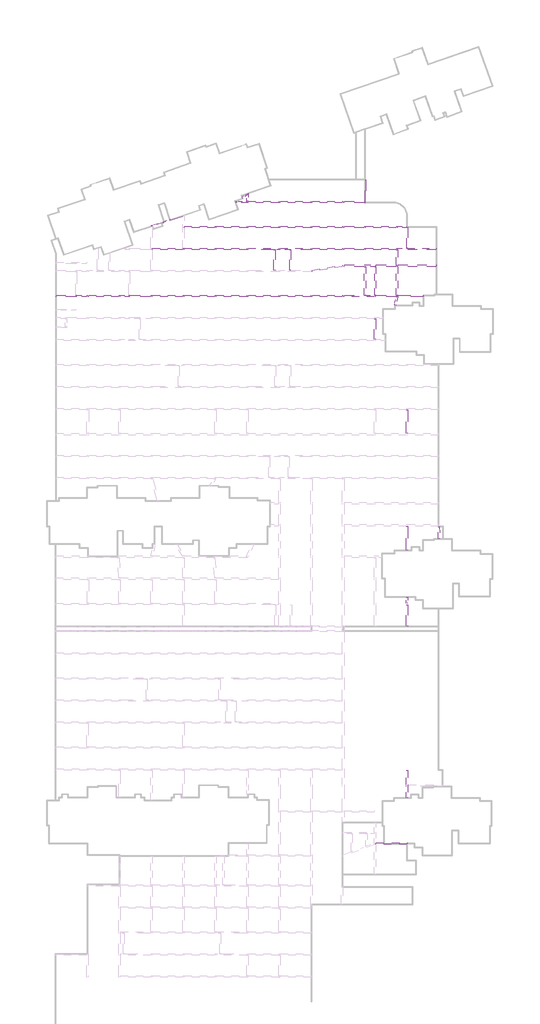
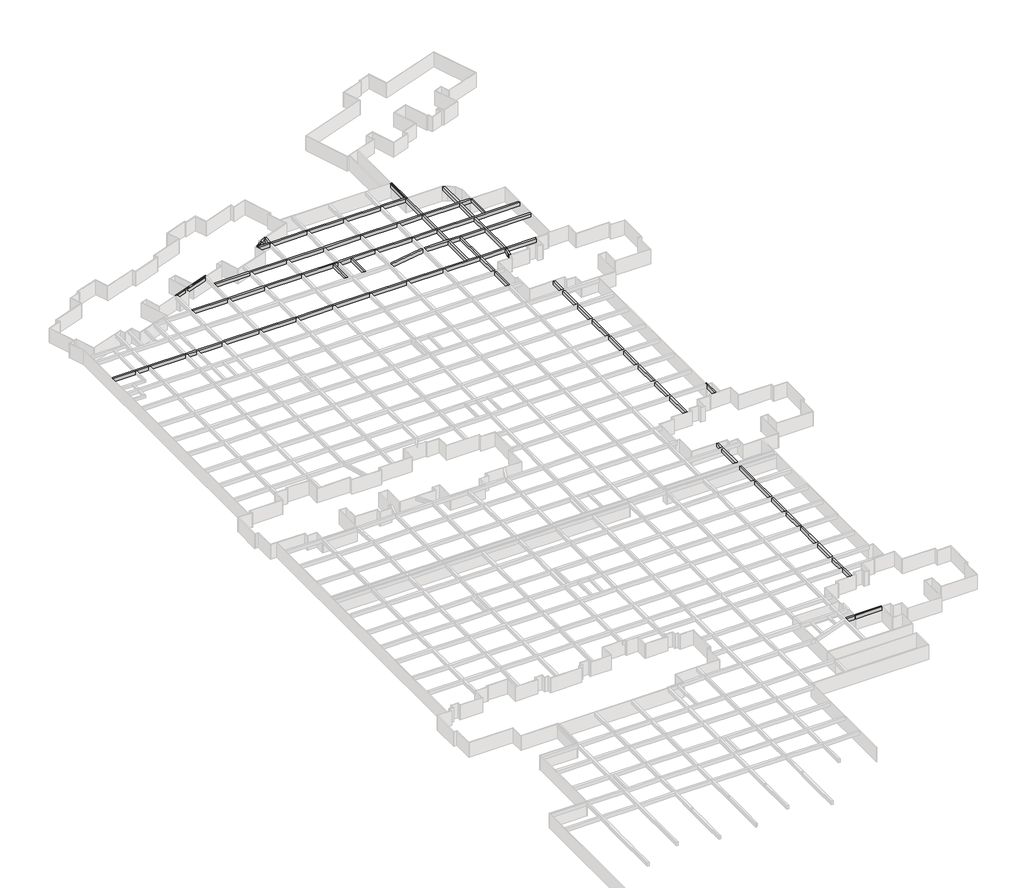
# One storey, part 14 of 14: 30 beams.
"""IFC4 building model written with IfcOpenShell, lengths in millimetres."""

from ifc_helpers import new_model, si_unit, frame, origin, place, context, project, spatial, polyline, outline, extrude, faceted_brep, element, save

model = new_model("IFC4")

# Units and contexts
model_context = context("Model", 3, world=origin())
ifc_project = project(units=[si_unit("LENGTHUNIT", "METRE", prefix="MILLI")], contexts=[model_context])

# Site, building, storey
site = spatial("IfcSite", under=ifc_project)
building = spatial("IfcBuilding", under=site)
storey = spatial("IfcBuildingStorey", under=building, Name="户型图", Elevation=0.0)

# Beams
placement = place(None, origin())
element("IfcBeam", 1, ObjectType="混凝土 - 矩形梁 : KL_beam", at=placement, inside=storey, context=model_context, shape_type="Brep", body=[
    faceted_brep([(-498755.1396851, -33759.4327531, 3300.0), (-498755.1396851, -33359.4327531, 3300.0), (-505917.6529954, -33359.4327531, 3300.0), (-506217.6529954, -33359.4327531, 3300.0), (-508367.954383, -33359.4327531, 3300.0), (-508767.954383, -33359.4327531, 3300.0), (-516417.6529954, -33359.4327531, 3300.0), (-516817.6529954, -33359.4327531, 3300.0), (-521867.6529954, -33359.4327531, 3300.0), (-522267.6529954, -33359.4327531, 3300.0), (-529867.6529954, -33359.4327531, 3300.0), (-530267.6529954, -33359.4327531, 3300.0), (-537867.6529954, -33359.4327531, 3300.0), (-538267.6529954, -33359.4327531, 3300.0), (-545867.6529954, -33359.4327531, 3300.0), (-546267.6529954, -33359.4327531, 3300.0), (-553867.6529954, -33359.4327531, 3300.0), (-554267.6529954, -33359.4327531, 3300.0), (-561867.6529954, -33359.4327531, 3300.0), (-562267.6529954, -33359.4327531, 3300.0), (-569867.6529954, -33359.4327531, 3300.0), (-569867.6529954, -33759.4327531, 3300.0), (-562267.6529954, -33759.4327531, 3300.0), (-561867.6529954, -33759.4327531, 3300.0), (-554267.6529954, -33759.4327531, 3300.0), (-553867.6529954, -33759.4327531, 3300.0), (-546267.6529954, -33759.4327531, 3300.0), (-545867.6529954, -33759.4327531, 3300.0), (-539417.6529954, -33759.4327531, 3300.0), (-539117.6529954, -33759.4327531, 3300.0), (-538267.6529954, -33759.4327531, 3300.0), (-537867.6529954, -33759.4327531, 3300.0), (-535517.6529954, -33759.4327531, 3300.0), (-535217.6529954, -33759.4327531, 3300.0), (-530267.6529954, -33759.4327531, 3300.0), (-529867.6529954, -33759.4327531, 3300.0), (-522267.6529954, -33759.4327531, 3300.0), (-521867.6529954, -33759.4327531, 3300.0), (-516817.6529954, -33759.4327531, 3300.0), (-516417.6529954, -33759.4327531, 3300.0), (-508767.954383, -33759.4327531, 3300.0), (-508367.954383, -33759.4327531, 3300.0), (-498755.1396851, -33759.4327531, 2500.0), (-569867.6529954, -33759.4327531, 2500.0), (-562267.6529954, -33759.4327531, 2500.0), (-561867.6529954, -33759.4327531, 2500.0), (-554267.6529954, -33759.4327531, 2500.0), (-553867.6529954, -33759.4327531, 2500.0), (-546267.6529954, -33759.4327531, 2500.0), (-545867.6529954, -33759.4327531, 2500.0), (-538267.6529954, -33759.4327531, 2500.0), (-537867.6529954, -33759.4327531, 2500.0), (-530267.6529954, -33759.4327531, 2500.0), (-529867.6529954, -33759.4327531, 2500.0), (-522267.6529954, -33759.4327531, 2500.0), (-521867.6529954, -33759.4327531, 2500.0), (-516817.6529954, -33759.4327531, 2500.0), (-516417.6529954, -33759.4327531, 2500.0), (-508767.954383, -33759.4327531, 2500.0), (-508367.954383, -33759.4327531, 2500.0), (-498755.1396851, -33359.4327531, 2500.0), (-569867.6529954, -33359.4327531, 2500.0), (-562267.6529954, -33359.4327531, 2500.0), (-561867.6529954, -33359.4327531, 2500.0), (-554267.6529954, -33359.4327531, 2500.0), (-553867.6529954, -33359.4327531, 2500.0), (-546267.6529954, -33359.4327531, 2500.0), (-545867.6529954, -33359.4327531, 2500.0), (-538267.6529954, -33359.4327531, 2500.0), (-537867.6529954, -33359.4327531, 2500.0), (-530267.6529954, -33359.4327531, 2500.0), (-529867.6529954, -33359.4327531, 2500.0), (-522267.6529954, -33359.4327531, 2500.0), (-521867.6529954, -33359.4327531, 2500.0), (-516817.6529954, -33359.4327531, 2500.0), (-516417.6529954, -33359.4327531, 2500.0), (-508767.954383, -33359.4327531, 2500.0), (-508367.954383, -33359.4327531, 2500.0)], [[[0, 1, 2, 3, 4, 5, 6, 7, 8, 9, 10, 11, 12, 13, 14, 15, 16, 17, 18, 19, 20, 21, 22, 23, 24, 25, 26, 27, 28, 29, 30, 31, 32, 33, 34, 35, 36, 37, 38, 39, 40, 41]], [[42, 0, 41, 40, 39, 38, 37, 36, 35, 34, 33, 32, 31, 30, 29, 28, 27, 26, 25, 24, 23, 22, 21, 43, 44, 45, 46, 47, 48, 49, 50, 51, 52, 53, 54, 55, 56, 57, 58, 59]], [[60, 42, 59, 58, 57, 56, 55, 54, 53, 52, 51, 50, 49, 48, 47, 46, 45, 44, 43, 61, 62, 63, 64, 65, 66, 67, 68, 69, 70, 71, 72, 73, 74, 75, 76, 77]], [[1, 60, 77, 76, 75, 74, 73, 72, 71, 70, 69, 68, 67, 66, 65, 64, 63, 62, 61, 20, 19, 18, 17, 16, 15, 14, 13, 12, 11, 10, 9, 8, 7, 6, 5, 4, 3, 2]], [[1, 0, 42, 60]], [[21, 20, 61, 43]]]),
])
element("IfcBeam", 2, ObjectType="混凝土 - 矩形梁 : KL_beam", at=placement, inside=storey, context=model_context, shape_type="Brep", body=[
    faceted_brep([(-506067.6529954, -28259.4327531, 3300.0), (-506067.6529954, -28059.4327531, 3300.0), (-506155.1396851, -28059.4327531, 3300.0), (-506155.1396851, -27939.4327531, 3300.0), (-506155.1396851, -27859.4327531, 3300.0), (-508367.954383, -27859.4327531, 3300.0), (-508767.954383, -27859.4327531, 3300.0), (-516417.6529954, -27859.4327531, 3300.0), (-516817.6529954, -27859.4327531, 3300.0), (-521867.6529954, -27859.4327531, 3300.0), (-522267.6529954, -27859.4327531, 3300.0), (-529867.6529954, -27859.4327531, 3300.0), (-530267.6529954, -27859.4327531, 3300.0), (-537867.6529954, -27859.4327531, 3300.0), (-538267.6529954, -27859.4327531, 3300.0), (-545867.6529954, -27859.4327531, 3300.0), (-546267.6529954, -27859.4327531, 3300.0), (-553867.6529954, -27859.4327531, 3300.0), (-554267.6529954, -27859.4327531, 3300.0), (-561867.6529954, -27859.4327531, 3300.0), (-561867.6529954, -28259.4327531, 3300.0), (-554267.6529954, -28259.4327531, 3300.0), (-553867.6529954, -28259.4327531, 3300.0), (-546267.6529954, -28259.4327531, 3300.0), (-545867.6529954, -28259.4327531, 3300.0), (-538267.6529954, -28259.4327531, 3300.0), (-537867.6529954, -28259.4327531, 3300.0), (-530267.6529954, -28259.4327531, 3300.0), (-529867.6529954, -28259.4327531, 3300.0), (-522267.6529954, -28259.4327531, 3300.0), (-521867.6529954, -28259.4327531, 3300.0), (-516817.6529954, -28259.4327531, 3300.0), (-516417.6529954, -28259.4327531, 3300.0), (-508767.954383, -28259.4327531, 3300.0), (-508367.954383, -28259.4327531, 3300.0), (-506217.6529954, -28259.4327531, 3300.0), (-506067.6529954, -28259.4327531, 2500.0), (-506067.6529954, -28259.4327531, 2700.0), (-561867.6529954, -28259.4327531, 2500.0), (-554267.6529954, -28259.4327531, 2500.0), (-553867.6529954, -28259.4327531, 2500.0), (-546267.6529954, -28259.4327531, 2500.0), (-545867.6529954, -28259.4327531, 2500.0), (-538267.6529954, -28259.4327531, 2500.0), (-537867.6529954, -28259.4327531, 2500.0), (-530267.6529954, -28259.4327531, 2500.0), (-529867.6529954, -28259.4327531, 2500.0), (-522267.6529954, -28259.4327531, 2500.0), (-521867.6529954, -28259.4327531, 2500.0), (-516817.6529954, -28259.4327531, 2500.0), (-516417.6529954, -28259.4327531, 2500.0), (-508767.954383, -28259.4327531, 2500.0), (-508367.954383, -28259.4327531, 2500.0), (-506067.6529954, -28059.4327531, 2500.0), (-561867.6529954, -27859.4327531, 2500.0), (-554267.6529954, -27859.4327531, 2500.0), (-553867.6529954, -27859.4327531, 2500.0), (-546267.6529954, -27859.4327531, 2500.0), (-545867.6529954, -27859.4327531, 2500.0), (-538267.6529954, -27859.4327531, 2500.0), (-537867.6529954, -27859.4327531, 2500.0), (-530267.6529954, -27859.4327531, 2500.0), (-529867.6529954, -27859.4327531, 2500.0), (-522267.6529954, -27859.4327531, 2500.0), (-521867.6529954, -27859.4327531, 2500.0), (-516817.6529954, -27859.4327531, 2500.0), (-516417.6529954, -27859.4327531, 2500.0), (-508767.954383, -27859.4327531, 2500.0), (-508367.954383, -27859.4327531, 2500.0), (-506155.1396851, -27859.4327531, 2500.0), (-506155.1396851, -28059.4327531, 2500.0), (-506067.6529954, -28059.4327531, 2700.0)], [[[0, 1, 2, 3, 4, 5, 6, 7, 8, 9, 10, 11, 12, 13, 14, 15, 16, 17, 18, 19, 20, 21, 22, 23, 24, 25, 26, 27, 28, 29, 30, 31, 32, 33, 34, 35]], [[36, 37, 0, 35, 34, 33, 32, 31, 30, 29, 28, 27, 26, 25, 24, 23, 22, 21, 20, 38, 39, 40, 41, 42, 43, 44, 45, 46, 47, 48, 49, 50, 51, 52]], [[53, 36, 52, 51, 50, 49, 48, 47, 46, 45, 44, 43, 42, 41, 40, 39, 38, 54, 55, 56, 57, 58, 59, 60, 61, 62, 63, 64, 65, 66, 67, 68, 69, 70]], [[4, 69, 68, 67, 66, 65, 64, 63, 62, 61, 60, 59, 58, 57, 56, 55, 54, 19, 18, 17, 16, 15, 14, 13, 12, 11, 10, 9, 8, 7, 6, 5]], [[70, 2, 1, 71, 53]], [[2, 70, 69, 4, 3]], [[0, 37, 36, 53, 71, 1]], [[20, 19, 54, 38]]]),
])
element("IfcBeam", 3, ObjectType="混凝土 - 矩形梁 : KL_beam", at=placement, inside=storey, context=model_context, shape_type="Brep", body=[
    faceted_brep([(-516677.6529954, -21959.2569935, 3300.0), (-516677.6529954, -21839.2569935, 3300.0), (-516677.6529954, -21559.4327531, 3300.0), (-516817.6529954, -21559.4327531, 3300.0), (-521867.6529954, -21559.4327531, 3300.0), (-522267.6529954, -21559.4327531, 3300.0), (-529867.6529954, -21559.4327531, 3300.0), (-530267.6529954, -21559.4327531, 3300.0), (-537867.6529954, -21559.4327531, 3300.0), (-538267.6529954, -21559.4327531, 3300.0), (-545867.6529954, -21559.4327531, 3300.0), (-546267.6529954, -21559.4327531, 3300.0), (-546267.6529954, -21959.4327531, 3300.0), (-545867.6529954, -21959.4327531, 3300.0), (-538267.6529954, -21959.4327531, 3300.0), (-537867.6529954, -21959.4327531, 3300.0), (-530267.6529954, -21959.4327531, 3300.0), (-529867.6529954, -21959.4327531, 3300.0), (-522267.6529954, -21959.4327531, 3300.0), (-521867.6529954, -21959.4327531, 3300.0), (-516817.6529954, -21959.4327531, 3300.0), (-516557.6529954, -21959.4327531, 3300.0), (-516557.6529954, -21959.2569935, 3300.0), (-516557.6529954, -21959.4327531, 2500.0), (-546267.6529954, -21959.4327531, 2500.0), (-545867.6529954, -21959.4327531, 2500.0), (-538267.6529954, -21959.4327531, 2500.0), (-537867.6529954, -21959.4327531, 2500.0), (-530267.6529954, -21959.4327531, 2500.0), (-529867.6529954, -21959.4327531, 2500.0), (-522267.6529954, -21959.4327531, 2500.0), (-521867.6529954, -21959.4327531, 2500.0), (-516817.6529954, -21959.4327531, 2500.0), (-516677.6529954, -21559.4327531, 2500.0), (-516677.6529954, -21959.2569935, 2500.0), (-516557.6529954, -21959.2569935, 2500.0), (-546267.6529954, -21559.4327531, 2500.0), (-545867.6529954, -21559.4327531, 2500.0), (-538267.6529954, -21559.4327531, 2500.0), (-537867.6529954, -21559.4327531, 2500.0), (-530267.6529954, -21559.4327531, 2500.0), (-529867.6529954, -21559.4327531, 2500.0), (-522267.6529954, -21559.4327531, 2500.0), (-521867.6529954, -21559.4327531, 2500.0), (-516817.6529954, -21559.4327531, 2500.0)], [[[0, 1, 2, 3, 4, 5, 6, 7, 8, 9, 10, 11, 12, 13, 14, 15, 16, 17, 18, 19, 20, 21, 22]], [[23, 21, 20, 19, 18, 17, 16, 15, 14, 13, 12, 24, 25, 26, 27, 28, 29, 30, 31, 32]], [[33, 34, 35, 23, 32, 31, 30, 29, 28, 27, 26, 25, 24, 36, 37, 38, 39, 40, 41, 42, 43, 44]], [[2, 33, 44, 43, 42, 41, 40, 39, 38, 37, 36, 11, 10, 9, 8, 7, 6, 5, 4, 3]], [[21, 23, 35, 22]], [[0, 34, 33, 2, 1]], [[34, 0, 22, 35]], [[12, 11, 36, 24]]]),
])
element("IfcBeam", 4, ObjectType="混凝土 - 矩形梁 : KL_beam", at=placement, inside=storey, context=model_context, shape_type="SweptSolid", body=[
    extrude(outline(polyline([(-529867.6529954, -39229.5561723), (-529867.6529954, -38824.309334), (-522267.6529954, -37589.309334), (-522267.6529954, -37994.5561723), (-529867.6529954, -39229.5561723)])), frame((0.0, 0.0, 2500.0), z_axis=(0.0, 0.0, 1.0), x_axis=(1.0, 0.0, 0.0)), (0.0, 0.0, 1.0), 800.0),
])
element("IfcBeam", 5, ObjectType="混凝土 - 矩形梁 : KL_beam", at=placement, inside=storey, context=model_context, shape_type="Brep", body=[
    faceted_brep([(-521867.6529954, -37559.4327532, 3300.0), (-521867.6529954, -37959.4327532, 3300.0), (-516817.6529954, -37959.4327532, 3300.0), (-516417.6529954, -37959.4327532, 3300.0), (-514217.6529954, -37959.4327532, 3300.0), (-513917.6529954, -37959.4327532, 3300.0), (-513917.6529954, -37559.4327532, 3300.0), (-516417.6529954, -37559.4327532, 3300.0), (-516817.6529954, -37559.4327532, 3300.0), (-513917.6529954, -37959.4327532, 2500.0), (-513917.6529954, -37959.4327532, 2700.0), (-521867.6529954, -37959.4327532, 2500.0), (-516817.6529954, -37959.4327532, 2500.0), (-516417.6529954, -37959.4327532, 2500.0), (-521867.6529954, -37559.4327532, 2500.0), (-516817.6529954, -37559.4327532, 2500.0), (-516417.6529954, -37559.4327532, 2500.0), (-513917.6529954, -37559.4327532, 2500.0)], [[[0, 1, 2, 3, 4, 5, 6, 7, 8]], [[9, 10, 5, 4, 3, 2, 1, 11, 12, 13]], [[11, 14, 15, 16, 17, 9, 13, 12]], [[14, 0, 8, 7, 6, 17, 16, 15]], [[0, 14, 11, 1]], [[6, 5, 10, 9, 17]]]),
])
element("IfcBeam", 6, ObjectType="混凝土 - 矩形梁 : KL_beam", at=placement, inside=storey, context=model_context, shape_type="SweptSolid", body=[
    extrude(outline(polyline([(-513917.6529954, -37959.4327532), (-513917.6529954, -37559.4327532), (-508767.954383, -37559.4327532), (-508767.954383, -37959.4327532), (-513917.6529954, -37959.4327532)])), frame((0.0, 0.0, 2500.0), z_axis=(0.0, 0.0, 1.0), x_axis=(1.0, 0.0, 0.0)), (0.0, 0.0, 1.0), 800.0),
])
element("IfcBeam", 7, ObjectType="混凝土 - 矩形梁 : KL_beam", at=placement, inside=storey, context=model_context, shape_type="SweptSolid", body=[
    extrude(outline(polyline([(-498755.1396851, -37559.4327532), (-498755.1396851, -37959.4327532), (-508367.954383, -37959.4327532), (-508367.954383, -37559.4327532), (-498755.1396851, -37559.4327532)])), frame((0.0, 0.0, 2500.0), z_axis=(0.0, 0.0, 1.0), x_axis=(1.0, 0.0, 0.0)), (0.0, 0.0, 1.0), 800.0),
])
element("IfcBeam", 8, ObjectType="混凝土 - 矩形梁 : KL_beam", at=placement, inside=storey, context=model_context, shape_type="Brep", body=[
    faceted_brep([(-508367.954383, -45559.4327531, 3300.0), (-508367.954383, -45159.4327531, 3300.0), (-508767.954383, -45159.4327531, 3300.0), (-513917.6529954, -45159.4327531, 3300.0), (-514217.6529954, -45159.4327531, 3300.0), (-516417.6529954, -45159.4327531, 3300.0), (-516817.6529954, -45159.4327531, 3300.0), (-521867.6529954, -45159.4327531, 3300.0), (-522267.6529954, -45159.4327531, 3300.0), (-529867.6529954, -45159.4327531, 3300.0), (-530267.6529954, -45159.4327531, 3300.0), (-537867.6529954, -45159.4327531, 3300.0), (-538267.6529954, -45159.4327531, 3300.0), (-545867.6529954, -45159.4327531, 3300.0), (-546267.6529954, -45159.4327531, 3300.0), (-553867.6529954, -45159.4327531, 3300.0), (-554267.6529954, -45159.4327531, 3300.0), (-561867.6529954, -45159.4327531, 3300.0), (-562267.6529954, -45159.4327531, 3300.0), (-569867.6529954, -45159.4327531, 3300.0), (-570267.6529954, -45159.4327531, 3300.0), (-575517.6529954, -45159.4327531, 3300.0), (-575817.6529954, -45159.4327531, 3300.0), (-577867.6529954, -45159.4327531, 3300.0), (-578267.6529954, -45159.4327531, 3300.0), (-585867.6529954, -45159.4327531, 3300.0), (-586267.6529954, -45159.4327531, 3300.0), (-588817.6529954, -45159.4327531, 3300.0), (-589117.6529954, -45159.4327531, 3300.0), (-594019.2557706, -45159.4327531, 3300.0), (-594019.2557706, -45559.4327531, 3300.0), (-589117.6529954, -45559.4327531, 3300.0), (-588817.6529954, -45559.4327531, 3300.0), (-586267.6529954, -45559.4327531, 3300.0), (-585867.6529954, -45559.4327531, 3300.0), (-578267.6529954, -45559.4327531, 3300.0), (-577867.6529954, -45559.4327531, 3300.0), (-575817.6529954, -45559.4327531, 3300.0), (-575517.6529954, -45559.4327531, 3300.0), (-570267.6529954, -45559.4327531, 3300.0), (-569867.6529954, -45559.4327531, 3300.0), (-562267.6529954, -45559.4327531, 3300.0), (-561867.6529954, -45559.4327531, 3300.0), (-554267.6529954, -45559.4327531, 3300.0), (-553867.6529954, -45559.4327531, 3300.0), (-546267.6529954, -45559.4327531, 3300.0), (-545867.6529954, -45559.4327531, 3300.0), (-538267.6529954, -45559.4327531, 3300.0), (-537867.6529954, -45559.4327531, 3300.0), (-530267.6529954, -45559.4327531, 3300.0), (-529867.6529954, -45559.4327531, 3300.0), (-522267.6529954, -45559.4327531, 3300.0), (-521867.6529954, -45559.4327531, 3300.0), (-514267.6529954, -45559.4327531, 3300.0), (-513867.6529954, -45559.4327531, 3300.0), (-508813.169158, -45559.4327531, 3300.0), (-508404.6952544, -45559.4327531, 3300.0), (-508367.954383, -45559.4327531, 2500.0), (-594019.2557706, -45559.4327531, 2500.0), (-586267.6529954, -45559.4327531, 2500.0), (-585867.6529954, -45559.4327531, 2500.0), (-578267.6529954, -45559.4327531, 2500.0), (-577867.6529954, -45559.4327531, 2500.0), (-570267.6529954, -45559.4327531, 2500.0), (-569867.6529954, -45559.4327531, 2500.0), (-562267.6529954, -45559.4327531, 2500.0), (-561867.6529954, -45559.4327531, 2500.0), (-554267.6529954, -45559.4327531, 2500.0), (-553867.6529954, -45559.4327531, 2500.0), (-546267.6529954, -45559.4327531, 2500.0), (-545867.6529954, -45559.4327531, 2500.0), (-538267.6529954, -45559.4327531, 2500.0), (-537867.6529954, -45559.4327531, 2500.0), (-530267.6529954, -45559.4327531, 2500.0), (-529867.6529954, -45559.4327531, 2500.0), (-522267.6529954, -45559.4327531, 2500.0), (-521867.6529954, -45559.4327531, 2500.0), (-514267.6529954, -45559.4327531, 2500.0), (-513867.6529954, -45559.4327531, 2500.0), (-508813.169158, -45559.4327531, 2500.0), (-508404.6952544, -45559.4327531, 2500.0), (-508367.954383, -45159.4327531, 2500.0), (-594019.2557706, -45159.4327531, 2500.0), (-586267.6529954, -45159.4327531, 2500.0), (-585867.6529954, -45159.4327531, 2500.0), (-578267.6529954, -45159.4327531, 2500.0), (-577867.6529954, -45159.4327531, 2500.0), (-570267.6529954, -45159.4327531, 2500.0), (-569867.6529954, -45159.4327531, 2500.0), (-562267.6529954, -45159.4327531, 2500.0), (-561867.6529954, -45159.4327531, 2500.0), (-554267.6529954, -45159.4327531, 2500.0), (-553867.6529954, -45159.4327531, 2500.0), (-546267.6529954, -45159.4327531, 2500.0), (-545867.6529954, -45159.4327531, 2500.0), (-538267.6529954, -45159.4327531, 2500.0), (-537867.6529954, -45159.4327531, 2500.0), (-530267.6529954, -45159.4327531, 2500.0), (-529867.6529954, -45159.4327531, 2500.0), (-522267.6529954, -45159.4327531, 2500.0), (-521867.6529954, -45159.4327531, 2500.0), (-516817.6529954, -45159.4327531, 2500.0), (-516417.6529954, -45159.4327531, 2500.0), (-508767.954383, -45159.4327531, 2500.0)], [[[0, 1, 2, 3, 4, 5, 6, 7, 8, 9, 10, 11, 12, 13, 14, 15, 16, 17, 18, 19, 20, 21, 22, 23, 24, 25, 26, 27, 28, 29, 30, 31, 32, 33, 34, 35, 36, 37, 38, 39, 40, 41, 42, 43, 44, 45, 46, 47, 48, 49, 50, 51, 52, 53, 54, 55, 56]], [[57, 0, 56, 55, 54, 53, 52, 51, 50, 49, 48, 47, 46, 45, 44, 43, 42, 41, 40, 39, 38, 37, 36, 35, 34, 33, 32, 31, 30, 58, 59, 60, 61, 62, 63, 64, 65, 66, 67, 68, 69, 70, 71, 72, 73, 74, 75, 76, 77, 78, 79, 80]], [[81, 57, 80, 79, 78, 77, 76, 75, 74, 73, 72, 71, 70, 69, 68, 67, 66, 65, 64, 63, 62, 61, 60, 59, 58, 82, 83, 84, 85, 86, 87, 88, 89, 90, 91, 92, 93, 94, 95, 96, 97, 98, 99, 100, 101, 102, 103]], [[1, 81, 103, 102, 101, 100, 99, 98, 97, 96, 95, 94, 93, 92, 91, 90, 89, 88, 87, 86, 85, 84, 83, 82, 29, 28, 27, 26, 25, 24, 23, 22, 21, 20, 19, 18, 17, 16, 15, 14, 13, 12, 11, 10, 9, 8, 7, 6, 5, 4, 3, 2]], [[30, 29, 82, 58]], [[1, 0, 57, 81]]]),
])
element("IfcBeam", 9, ObjectType="混凝土 - 矩形梁 : KL_beam", at=placement, inside=storey, context=model_context, shape_type="Brep", body=[
    faceted_brep([(-502015.1396851, -45559.4327531, 3300.0), (-502015.1396851, -45292.3075196, 3300.0), (-502015.1396851, -45172.3075196, 3300.0), (-501895.1396851, -45172.3075196, 3300.0), (-501895.1396851, -45159.4327531, 3300.0), (-508367.954383, -45159.4327531, 3300.0), (-508367.954383, -45559.4327531, 3300.0), (-502015.1396851, -45559.4327531, 2500.0), (-508367.954383, -45559.4327531, 2500.0), (-502015.1396851, -45172.3075196, 2500.0), (-508367.954383, -45159.4327531, 2500.0), (-501895.1396851, -45159.4327531, 2500.0), (-501895.1396851, -45172.3075196, 2500.0)], [[[0, 1, 2, 3, 4, 5, 6]], [[7, 0, 6, 8]], [[9, 7, 8, 10, 11, 12]], [[4, 11, 10, 5]], [[11, 4, 3, 12]], [[0, 7, 9, 2, 1]], [[2, 9, 12, 3]], [[6, 5, 10, 8]]]),
])
element("IfcBeam", 10, ObjectType="混凝土 - 矩形梁 : KL_beam", at=placement, inside=storey, context=model_context, shape_type="Brep", body=[
    faceted_brep([(-567194.1270285, -27105.5852075, 2500.0), (-567194.1270285, -27105.5852075, 3300.0), (-567238.9034733, -26972.9387979, 3300.0), (-567238.9034733, -26972.9387979, 2500.0), (-562267.6529954, -25442.5926439, 2500.0), (-562267.6529954, -25442.5926439, 3300.0), (-562267.6529954, -25294.8313886, 2500.0), (-562267.6529954, -25294.8313886, 3300.0), (-566850.6148569, -26841.8671476, 3300.0), (-566850.6148569, -26841.8671476, 2500.0), (-566888.9946667, -26728.170225, 3300.0), (-566933.7711116, -26595.5238154, 3300.0), (-566933.7711116, -26595.5238154, 2500.0), (-565497.231347, -26385.0157164, 3300.0), (-565497.231347, -26385.0157164, 2500.0), (-565580.3876017, -26138.6723843, 2500.0), (-565580.3876017, -26138.6723843, 3300.0), (-565383.5344245, -26346.6359066, 3300.0)], [[[0, 1, 2, 3]], [[1, 0, 4, 5]], [[5, 4, 6, 7]], [[8, 9, 3, 2]], [[9, 8, 10, 11, 12]], [[13, 14, 15, 16]], [[14, 13, 17, 7, 6]], [[12, 11, 16, 15]], [[1, 5, 7, 17, 13, 16, 11, 10, 8, 2]], [[4, 0, 3, 9, 12, 15, 14, 6]]]),
    faceted_brep([(-565421.9142343, -26232.938984, 3300.0), (-561948.5420308, -25060.4590103, 3300.0), (-561993.3184757, -24927.8126006, 3300.0), (-565466.6906792, -26100.2925744, 3300.0), (-561993.3184757, -24927.8126006, 2500.0), (-561948.5420308, -25060.4590103, 2500.0), (-565421.9142343, -26232.938984, 2500.0), (-565466.6906792, -26100.2925744, 2500.0)], [[[0, 1, 2, 3]], [[4, 5, 6, 7]], [[2, 4, 7, 3]], [[4, 2, 1, 5]], [[0, 6, 5, 1]], [[3, 7, 6, 0]]]),
    faceted_brep([(-567277.2832832, -26859.2418753, 3300.0), (-567277.2832832, -26859.2418753, 2500.0), (-567002.6915893, -26766.5500349, 2500.0), (-567002.6915893, -26766.5500349, 3300.0), (-567322.059728, -26726.5954657, 3300.0), (-567322.059728, -26726.5954657, 2500.0), (-567047.4680341, -26633.9036253, 3300.0), (-567047.4680341, -26633.9036253, 2500.0)], [[[0, 1, 2, 3]], [[4, 5, 1, 0]], [[6, 3, 2, 7]], [[4, 0, 3, 6]], [[1, 5, 7, 2]], [[5, 4, 6, 7]]]),
])
element("IfcBeam", 11, ObjectType="混凝土 - 矩形梁 : KL_beam", at=placement, inside=storey, context=model_context, shape_type="SweptSolid", body=[
    extrude(outline(polyline([(-570131.0843915, -27668.6081906), (-566657.7255059, -26503.8089794), (-566575.5004889, -26748.998872), (-566850.6148569, -26841.8671476), (-566888.9946667, -26728.170225), (-567665.8108881, -26990.3941992), (-567627.6568009, -27104.1673172), (-569867.6529954, -27860.3058838), (-569867.6529954, -27798.4711532), (-570060.5174914, -27798.4711532), (-570084.8033221, -27806.6154647), (-570131.0843915, -27668.6081906)])), frame((0.0, 0.0, 2500.0), z_axis=(0.0, 0.0, 1.0), x_axis=(1.0, 0.0, 0.0)), (0.0, 0.0, 1.0), 800.0),
])
element("IfcBeam", 12, ObjectType="混凝土 - 矩形梁 : KL_beam", at=placement, inside=storey, context=model_context, shape_type="Brep", body=[
    faceted_brep([(-546179.2460997, -19597.0204925, 2500.0), (-546179.2460997, -19597.0204925, 3300.0), (-546161.9464573, -19622.8510562, 3300.0), (-546161.9464573, -19622.8510562, 2500.0), (-546273.8443347, -19660.3762771, 3300.0), (-546273.8443347, -19660.3762771, 2500.0)], [[[0, 1, 2, 3]], [[2, 1, 4]], [[0, 3, 5]], [[1, 0, 5, 4]], [[3, 2, 4, 5]]]),
    faceted_brep([(-548829.2329536, -21853.2325756, 2500.0), (-548829.2329536, -21853.2325756, 3300.0), (-549026.0010884, -21559.4327531, 3300.0), (-549029.1521409, -21554.7278314, 3300.0), (-549029.1521409, -21554.7278314, 2500.0), (-549026.0010884, -21559.4327531, 2500.0), (-548390.5524947, -21559.4327531, 2500.0), (-547736.0310301, -21121.0765735, 2500.0), (-547736.0310301, -21121.0765735, 3300.0), (-548390.5524947, -21559.4327531, 3300.0)], [[[0, 1, 2, 3, 4, 5]], [[1, 0, 6, 7, 8, 9]], [[4, 3, 8, 7]], [[3, 2, 1, 9, 8]], [[0, 5, 4, 7, 6]]]),
    faceted_brep([(-545956.6604485, -19929.3691466, 2500.0), (-545956.6604485, -19929.3691466, 3300.0), (-546267.6529954, -20137.6518572, 3300.0), (-547255.5675769, -20799.2932016, 3300.0), (-547255.5675769, -20799.2932016, 2500.0), (-546267.6529954, -20137.6518572, 2500.0), (-547388.1122393, -20406.640912, 3300.0), (-547388.1122393, -20406.640912, 2500.0), (-546092.7261364, -19726.205789, 3300.0), (-546092.7261364, -19726.205789, 2500.0), (-546652.3562174, -19913.8790754, 2500.0), (-546652.3562174, -19913.8790754, 3300.0)], [[[0, 1, 2, 3, 4, 5]], [[3, 6, 7, 4]], [[8, 9, 10, 11]], [[1, 0, 9, 8]], [[3, 2, 1, 8, 11, 6]], [[0, 5, 4, 7, 10, 9]], [[7, 6, 11, 10]]]),
    faceted_brep([(-547491.4111778, -20475.8238654, 3300.0), (-547359.0031341, -20868.0714336, 3300.0), (-547359.0031341, -20868.0714336, 2500.0), (-547491.4111778, -20475.8238654, 2500.0), (-548797.2519129, -21350.3916022, 3300.0), (-548797.2519129, -21350.3916022, 2500.0)], [[[0, 1, 2, 3]], [[1, 0, 4]], [[3, 2, 5]], [[0, 3, 5, 4]], [[2, 1, 4, 5]]]),
])
element("IfcBeam", 13, ObjectType="混凝土 - 矩形梁 : KL_beam", at=placement, inside=storey, context=model_context, shape_type="SweptSolid", body=[
    extrude(outline(polyline([(-516417.6529954, -21959.4327531), (-516557.6529954, -21959.4327531), (-516557.6529954, -21959.2569935), (-516417.6529954, -21959.2569935), (-516417.6529954, -21959.4327531)])), frame((0.0, 0.0, 2500.0), z_axis=(0.0, 0.0, 1.0), x_axis=(1.0, 0.0, 0.0)), (0.0, 0.0, 1.0), 800.0),
    extrude(outline(polyline([(-516817.6529954, -16219.4327531), (-516677.6529954, -16219.4327531), (-516677.6529954, -21559.4327531), (-516817.6529954, -21559.4327531), (-516817.6529954, -16219.4327531)])), frame((0.0, 0.0, 2500.0), z_axis=(0.0, 0.0, 1.0), x_axis=(1.0, 0.0, 0.0)), (0.0, 0.0, 1.0), 800.0),
    extrude(outline(polyline([(-516417.6529954, -16159.4327531), (-516417.6529954, -21839.2569935), (-516557.6529954, -21839.2569935), (-516557.6529954, -16159.4327531), (-516417.6529954, -16159.4327531)])), frame((0.0, 0.0, 2500.0), z_axis=(0.0, 0.0, 1.0), x_axis=(1.0, 0.0, 0.0)), (0.0, 0.0, 1.0), 800.0),
])
element("IfcBeam", 14, ObjectType="混凝土 - 矩形梁 : KL_beam", at=placement, inside=storey, context=model_context, shape_type="Brep", body=[
    faceted_brep([(-516817.6529954, -45159.4327531, 3300.0), (-516417.6529954, -45159.4327531, 3300.0), (-516417.6529954, -37959.4327532, 3300.0), (-516817.6529954, -37959.4327532, 3300.0), (-516817.6529954, -45159.4327531, 2500.0), (-516817.6529954, -37959.4327532, 2500.0), (-516417.6529954, -45159.4327531, 2500.0), (-516417.6529954, -37959.4327532, 2500.0)], [[[0, 1, 2, 3]], [[4, 0, 3, 5]], [[6, 4, 5, 7]], [[1, 6, 7, 2]], [[1, 0, 4, 6]], [[3, 2, 7, 5]]]),
    faceted_brep([(-516817.6529954, -21959.4327531, 2500.0), (-516817.6529954, -21959.4327531, 3300.0), (-516557.6529954, -21959.4327531, 3300.0), (-516417.6529954, -21959.4327531, 3300.0), (-516417.6529954, -21959.4327531, 2500.0), (-516557.6529954, -21959.4327531, 2500.0), (-516417.6529954, -27859.4327531, 3300.0), (-516817.6529954, -27859.4327531, 3300.0), (-516817.6529954, -27859.4327531, 2500.0), (-516417.6529954, -27859.4327531, 2500.0)], [[[0, 1, 2, 3, 4, 5]], [[6, 7, 8, 9]], [[3, 2, 1, 7, 6]], [[1, 0, 8, 7]], [[0, 5, 4, 9, 8]], [[4, 3, 6, 9]]]),
    faceted_brep([(-516817.6529954, -33759.4327531, 3300.0), (-516417.6529954, -33759.4327531, 3300.0), (-516417.6529954, -33759.4327531, 2500.0), (-516817.6529954, -33759.4327531, 2500.0), (-516417.6529954, -37559.4327532, 3300.0), (-516817.6529954, -37559.4327532, 3300.0), (-516817.6529954, -37559.4327532, 2500.0), (-516417.6529954, -37559.4327532, 2500.0)], [[[0, 1, 2, 3]], [[4, 5, 6, 7]], [[1, 0, 5, 4]], [[0, 3, 6, 5]], [[3, 2, 7, 6]], [[2, 1, 4, 7]]]),
    faceted_brep([(-516417.6529954, -33359.4327531, 3300.0), (-516817.6529954, -33359.4327531, 3300.0), (-516817.6529954, -33359.4327531, 2500.0), (-516417.6529954, -33359.4327531, 2500.0), (-516417.6529954, -28259.4327531, 3300.0), (-516817.6529954, -28259.4327531, 3300.0), (-516817.6529954, -28259.4327531, 2500.0), (-516417.6529954, -28259.4327531, 2500.0)], [[[0, 1, 2, 3]], [[1, 0, 4, 5]], [[2, 1, 5, 6]], [[3, 2, 6, 7]], [[0, 3, 7, 4]], [[5, 4, 7, 6]]]),
])
element("IfcBeam", 15, ObjectType="混凝土 - 矩形梁 : KL_beam", at=placement, inside=storey, context=model_context, shape_type="Brep", body=[
    faceted_brep([(-508367.954383, -22175.1198686, 3300.0), (-508767.954383, -22021.1648556, 3300.0), (-508767.954383, -27859.4327531, 3300.0), (-508367.954383, -27859.4327531, 3300.0), (-508367.954383, -22175.1198686, 2500.0), (-508367.954383, -27859.4327531, 2500.0), (-508767.954383, -22021.1648556, 2500.0), (-508767.954383, -27859.4327531, 2500.0)], [[[0, 1, 2, 3]], [[4, 0, 3, 5]], [[6, 4, 5, 7]], [[1, 6, 7, 2]], [[1, 0, 4, 6]], [[3, 2, 7, 5]]]),
    faceted_brep([(-508367.954383, -45159.4327531, 3300.0), (-508767.954383, -45159.4327531, 3300.0), (-508767.954383, -45159.4327531, 2500.0), (-508367.954383, -45159.4327531, 2500.0), (-508767.954383, -33759.4327531, 3300.0), (-508367.954383, -33759.4327531, 3300.0), (-508367.954383, -33759.4327531, 2500.0), (-508767.954383, -33759.4327531, 2500.0), (-508367.954383, -37959.4327532, 3300.0), (-508367.954383, -37559.4327532, 3300.0), (-508767.954383, -37559.4327532, 3300.0), (-508767.954383, -37959.4327532, 3300.0), (-508367.954383, -37959.4327532, 2500.0), (-508367.954383, -37559.4327532, 2500.0), (-508767.954383, -37959.4327532, 2500.0), (-508767.954383, -37559.4327532, 2500.0)], [[[0, 1, 2, 3]], [[4, 5, 6, 7]], [[1, 0, 8, 9, 5, 4, 10, 11]], [[0, 3, 12, 13, 6, 5, 9, 8]], [[3, 2, 14, 15, 7, 6, 13, 12]], [[2, 1, 11, 10, 4, 7, 15, 14]]]),
    faceted_brep([(-508367.954383, -33359.4327531, 3300.0), (-508767.954383, -33359.4327531, 3300.0), (-508767.954383, -33359.4327531, 2500.0), (-508367.954383, -33359.4327531, 2500.0), (-508767.954383, -28259.4327531, 3300.0), (-508367.954383, -28259.4327531, 3300.0), (-508367.954383, -28259.4327531, 2500.0), (-508767.954383, -28259.4327531, 2500.0)], [[[0, 1, 2, 3]], [[4, 5, 6, 7]], [[1, 0, 5, 4]], [[0, 3, 6, 5]], [[3, 2, 7, 6]], [[2, 1, 4, 7]]]),
])
element("IfcBeam", 16, ObjectType="混凝土 - 矩形梁 : KL_beam", at=placement, inside=storey, context=model_context, shape_type="SweptSolid", body=[
    extrude(outline(polyline([(-514267.6529954, -45559.4327531), (-513867.6529954, -45559.4327531), (-513867.6529954, -50659.4327531), (-514267.6529954, -50659.4327531), (-514267.6529954, -45559.4327531)])), frame((0.0, 0.0, 2500.0), z_axis=(0.0, 0.0, 1.0), x_axis=(1.0, 0.0, 0.0)), (0.0, 0.0, 1.0), 800.0),
    extrude(outline(polyline([(-513867.6529954, -56159.4327531), (-514267.6529954, -56159.4327531), (-514267.6529954, -51059.4327531), (-513867.6529954, -51059.4327531), (-513867.6529954, -56159.4327531)])), frame((0.0, 0.0, 2500.0), z_axis=(0.0, 0.0, 1.0), x_axis=(1.0, 0.0, 0.0)), (0.0, 0.0, 1.0), 800.0),
])
element("IfcBeam", 17, ObjectType="混凝土 - 矩形梁 : KL_beam", at=placement, inside=storey, context=model_context, shape_type="SweptSolid", body=[
    extrude(outline(polyline([(-506267.6529954, -59259.003002), (-505867.6529954, -59259.003002), (-505867.6529954, -62459.4327531), (-506267.6529954, -62459.4327531), (-506267.6529954, -59259.003002)])), frame((0.0, 0.0, 2500.0), z_axis=(0.0, 0.0, 1.0), x_axis=(1.0, 0.0, 0.0)), (0.0, 0.0, 1.0), 800.0),
    extrude(outline(polyline([(-505867.6529954, -90759.4327531), (-506267.6529954, -90759.4327531), (-506267.6529954, -85659.4327531), (-505867.6529954, -85659.4327531), (-505867.6529954, -90759.4327531)])), frame((0.0, 0.0, 2500.0), z_axis=(0.0, 0.0, 1.0), x_axis=(1.0, 0.0, 0.0)), (0.0, 0.0, 1.0), 800.0),
    extrude(outline(polyline([(-506267.6529954, -62859.4327531), (-505867.6529954, -62859.4327531), (-505867.6529954, -67959.4327531), (-506267.6529954, -67959.4327531), (-506267.6529954, -62859.4327531)])), frame((0.0, 0.0, 2500.0), z_axis=(0.0, 0.0, 1.0), x_axis=(1.0, 0.0, 0.0)), (0.0, 0.0, 1.0), 800.0),
    extrude(outline(polyline([(-506267.6529954, -68359.4327531), (-505867.6529954, -68359.4327531), (-505867.6529954, -73459.4327531), (-506267.6529954, -73459.4327531), (-506267.6529954, -68359.4327531)])), frame((0.0, 0.0, 2500.0), z_axis=(0.0, 0.0, 1.0), x_axis=(1.0, 0.0, 0.0)), (0.0, 0.0, 1.0), 800.0),
    extrude(outline(polyline([(-506267.6529954, -73859.4327531), (-505867.6529954, -73859.4327531), (-505867.6529954, -79759.4327531), (-506267.6529954, -79759.4327531), (-506267.6529954, -73859.4327531)])), frame((0.0, 0.0, 2500.0), z_axis=(0.0, 0.0, 1.0), x_axis=(1.0, 0.0, 0.0)), (0.0, 0.0, 1.0), 800.0),
    extrude(outline(polyline([(-506267.6529954, -80159.4327531), (-505867.6529954, -80159.4327531), (-505867.6529954, -85259.4327531), (-506267.6529954, -85259.4327531), (-506267.6529954, -80159.4327531)])), frame((0.0, 0.0, 2500.0), z_axis=(0.0, 0.0, 1.0), x_axis=(1.0, 0.0, 0.0)), (0.0, 0.0, 1.0), 800.0),
])
element("IfcBeam", 18, ObjectType="混凝土 - 矩形梁 : KL_beam", at=placement, inside=storey, context=model_context, shape_type="SweptSolid", body=[
    extrude(outline(polyline([(-509115.1396851, -47655.7967618), (-509115.1396851, -47018.750239), (-508813.169158, -45559.4327531), (-508404.6952544, -45559.4327531), (-508838.4871816, -47655.7967618), (-509115.1396851, -47655.7967618)])), frame((0.0, 0.0, 2500.0), z_axis=(0.0, 0.0, 1.0), x_axis=(1.0, 0.0, 0.0)), (0.0, 0.0, 1.0), 800.0),
])
element("IfcBeam", 19, ObjectType="混凝土 - 矩形梁 : KL_beam", at=placement, inside=storey, context=model_context, shape_type="SweptSolid", body=[
    extrude(outline(polyline([(-505867.6529954, -108997.5126628), (-506267.6529954, -108997.5126628), (-506267.6529954, -102959.4327531), (-505867.6529954, -102959.4327531), (-505867.6529954, -108997.5126628)])), frame((0.0, 0.0, 2500.0), z_axis=(0.0, 0.0, 1.0), x_axis=(1.0, 0.0, 0.0)), (0.0, 0.0, 1.0), 800.0),
    extrude(outline(polyline([(-506267.6529954, -91159.4327531), (-505867.6529954, -91159.4327531), (-505867.6529954, -97059.4327531), (-506267.6529954, -97059.4327531), (-506267.6529954, -91159.4327531)])), frame((0.0, 0.0, 2500.0), z_axis=(0.0, 0.0, 1.0), x_axis=(1.0, 0.0, 0.0)), (0.0, 0.0, 1.0), 800.0),
    extrude(outline(polyline([(-506267.6529954, -97459.4327531), (-505867.6529954, -97459.4327531), (-505867.6529954, -102559.4327531), (-506267.6529954, -102559.4327531), (-506267.6529954, -97459.4327531)])), frame((0.0, 0.0, 2500.0), z_axis=(0.0, 0.0, 1.0), x_axis=(1.0, 0.0, 0.0)), (0.0, 0.0, 1.0), 800.0),
])
element("IfcBeam", 20, ObjectType="混凝土 - 矩形梁 : KL_beam", at=placement, inside=storey, context=model_context, shape_type="Brep", body=[
    faceted_brep([(-498277.6529954, -105969.2261541, 3300.0), (-498270.4642181, -106133.8197785, 3300.0), (-497870.0828827, -106133.8197785, 3300.0), (-498000.237113, -103153.8197785, 3300.0), (-498277.6529954, -103153.8197785, 3300.0), (-498277.6529954, -105969.2261541, 2500.0), (-498270.4642181, -106133.8197785, 2500.0), (-498277.6529954, -103153.8197785, 2500.0), (-498000.237113, -103153.8197785, 2500.0), (-497870.0828827, -106133.8197785, 2500.0)], [[[0, 1, 2, 3, 4]], [[0, 5, 6, 1]], [[6, 5, 7, 8, 9]], [[2, 9, 8, 3]], [[5, 0, 4, 7]], [[2, 1, 6, 9]], [[4, 3, 8, 7]]]),
    faceted_brep([(-498157.6529954, -102959.4327531, 3300.0), (-498157.6529954, -102559.4327531, 3300.0), (-498157.6529954, -102559.4327531, 2500.0), (-498157.6529954, -102959.4327531, 2500.0), (-498157.6529954, -103033.8197785, 2500.0), (-498157.6529954, -103033.8197785, 3300.0), (-498005.478223, -103033.8197785, 3300.0), (-498005.478223, -103033.8197785, 2500.0), (-498026.197511, -102559.4327531, 3300.0), (-498026.197511, -102559.4327531, 2500.0)], [[[0, 1, 2, 3, 4, 5]], [[6, 5, 4, 7]], [[1, 0, 5, 6, 8]], [[4, 3, 2, 9, 7]], [[9, 8, 6, 7]], [[8, 9, 2, 1]]]),
])
element("IfcBeam", 21, ObjectType="混凝土 - 矩形梁 : KL_beam", at=placement, inside=storey, context=model_context, shape_type="SweptSolid", body=[
    extrude(outline(polyline([(-506267.6529954, -120740.3535812), (-505867.6529954, -120740.3535812), (-505867.6529954, -122259.4327531), (-506267.6529954, -122259.4327531), (-506267.6529954, -120740.3535812)])), frame((0.0, 0.0, 2500.0), z_axis=(0.0, 0.0, 1.0), x_axis=(1.0, 0.0, 0.0)), (0.0, 0.0, 1.0), 800.0),
])
element("IfcBeam", 22, ObjectType="混凝土 - 矩形梁 : KL_beam", at=placement, inside=storey, context=model_context, shape_type="Brep", body=[
    faceted_brep([(-506267.6529954, -128099.4327532, 3300.0), (-505867.6529954, -128099.4327532, 3300.0), (-505867.6529954, -127959.4327532, 3300.0), (-505867.6529954, -122659.4327531, 3300.0), (-506267.6529954, -122659.4327531, 3300.0), (-506267.6529954, -127959.4327532, 3300.0), (-505867.6529954, -128099.4327532, 2500.0), (-505867.6529954, -127959.4327532, 2500.0), (-505867.6529954, -122659.4327531, 2500.0), (-506267.6529954, -128099.4327532, 2500.0), (-506267.6529954, -127959.4327532, 2500.0), (-506267.6529954, -122659.4327531, 2500.0)], [[[0, 1, 2, 3, 4, 5]], [[1, 6, 7, 8, 3, 2]], [[6, 9, 10, 11, 8, 7]], [[9, 0, 5, 4, 11, 10]], [[1, 0, 9, 6]], [[4, 3, 8, 11]]]),
])
element("IfcBeam", 23, ObjectType="混凝土 - 矩形梁 : KL_beam", at=placement, inside=storey, context=model_context, shape_type="Brep", body=[
    faceted_brep([(-506267.6529954, -171018.3612758, 3300.0), (-505867.6529954, -171018.3612758, 3300.0), (-505867.6529954, -168200.507479, 3300.0), (-505867.6529954, -167800.507479, 3300.0), (-505867.6529954, -164159.4327531, 3300.0), (-506267.6529954, -164159.4327531, 3300.0), (-506267.6529954, -167800.507479, 3300.0), (-506267.6529954, -168200.507479, 3300.0), (-505867.6529954, -171018.3612758, 2500.0), (-505867.6529954, -168200.507479, 2500.0), (-505867.6529954, -167800.507479, 2500.0), (-505867.6529954, -164159.4327531, 2500.0), (-506267.6529954, -171018.3612758, 2500.0), (-506267.6529954, -168200.507479, 2500.0), (-506267.6529954, -167800.507479, 2500.0), (-506267.6529954, -164159.4327531, 2500.0)], [[[0, 1, 2, 3, 4, 5, 6, 7]], [[1, 8, 9, 10, 11, 4, 3, 2]], [[8, 12, 13, 14, 15, 11, 10, 9]], [[12, 0, 7, 6, 5, 15, 14, 13]], [[1, 0, 12, 8]], [[5, 4, 11, 15]]]),
    faceted_brep([(-506267.6529954, -129434.4327531, 3300.0), (-505867.6529954, -129434.4327531, 3300.0), (-505867.6529954, -129434.4327531, 2500.0), (-506267.6529954, -129434.4327531, 2500.0), (-505867.6529954, -134659.4327531, 3300.0), (-506267.6529954, -134659.4327531, 3300.0), (-506267.6529954, -134659.4327531, 2500.0), (-505867.6529954, -134659.4327531, 2500.0)], [[[0, 1, 2, 3]], [[4, 5, 6, 7]], [[1, 0, 5, 4]], [[2, 1, 4, 7]], [[3, 2, 7, 6]], [[0, 3, 6, 5]]]),
    faceted_brep([(-506267.6529954, -135059.4327531, 3300.0), (-505867.6529954, -135059.4327531, 3300.0), (-505867.6529954, -135059.4327531, 2500.0), (-506267.6529954, -135059.4327531, 2500.0), (-505867.6529954, -140959.4327531, 3300.0), (-506267.6529954, -140959.4327531, 3300.0), (-506267.6529954, -140959.4327531, 2500.0), (-505867.6529954, -140959.4327531, 2500.0)], [[[0, 1, 2, 3]], [[4, 5, 6, 7]], [[1, 0, 5, 4]], [[2, 1, 4, 7]], [[3, 2, 7, 6]], [[0, 3, 6, 5]]]),
    faceted_brep([(-506267.6529954, -141359.4327531, 3300.0), (-505867.6529954, -141359.4327531, 3300.0), (-505867.6529954, -141359.4327531, 2500.0), (-506267.6529954, -141359.4327531, 2500.0), (-505867.6529954, -146459.4327531, 3300.0), (-506267.6529954, -146459.4327531, 3300.0), (-506267.6529954, -146459.4327531, 2500.0), (-505867.6529954, -146459.4327531, 2500.0)], [[[0, 1, 2, 3]], [[4, 5, 6, 7]], [[1, 0, 5, 4]], [[2, 1, 4, 7]], [[3, 2, 7, 6]], [[0, 3, 6, 5]]]),
    faceted_brep([(-506267.6529954, -146859.4327531, 3300.0), (-505867.6529954, -146859.4327531, 3300.0), (-505867.6529954, -146859.4327531, 2500.0), (-506267.6529954, -146859.4327531, 2500.0), (-505867.6529954, -151959.4327531, 3300.0), (-506267.6529954, -151959.4327531, 3300.0), (-506267.6529954, -151959.4327531, 2500.0), (-505867.6529954, -151959.4327531, 2500.0)], [[[0, 1, 2, 3]], [[4, 5, 6, 7]], [[1, 0, 5, 4]], [[2, 1, 4, 7]], [[3, 2, 7, 6]], [[0, 3, 6, 5]]]),
    faceted_brep([(-506267.6529954, -152359.4327531, 3300.0), (-505867.6529954, -152359.4327531, 3300.0), (-505867.6529954, -152359.4327531, 2500.0), (-506267.6529954, -152359.4327531, 2500.0), (-505867.6529954, -158259.4327531, 3300.0), (-506267.6529954, -158259.4327531, 3300.0), (-506267.6529954, -158259.4327531, 2500.0), (-505867.6529954, -158259.4327531, 2500.0)], [[[0, 1, 2, 3]], [[4, 5, 6, 7]], [[1, 0, 5, 4]], [[2, 1, 4, 7]], [[3, 2, 7, 6]], [[0, 3, 6, 5]]]),
    faceted_brep([(-506267.6529954, -158659.4327531, 3300.0), (-505867.6529954, -158659.4327531, 3300.0), (-505867.6529954, -158659.4327531, 2500.0), (-506267.6529954, -158659.4327531, 2500.0), (-505867.6529954, -163759.4327531, 3300.0), (-506267.6529954, -163759.4327531, 3300.0), (-506267.6529954, -163759.4327531, 2500.0), (-505867.6529954, -163759.4327531, 2500.0)], [[[0, 1, 2, 3]], [[4, 5, 6, 7]], [[1, 0, 5, 4]], [[2, 1, 4, 7]], [[3, 2, 7, 6]], [[0, 3, 6, 5]]]),
])
element("IfcBeam", 24, ObjectType="混凝土 - 矩形梁 : KL_beam", at=placement, inside=storey, context=model_context, shape_type="SweptSolid", body=[
    extrude(outline(polyline([(-506007.6529952, -182324.2232736), (-506007.6529952, -182464.2232736), (-506127.6529952, -182464.2232736), (-506127.6529952, -182724.2232736), (-513867.6529954, -182724.2232736), (-513867.6529954, -182324.2232736), (-506007.6529952, -182324.2232736)])), frame((0.0, 0.0, 2500.0), z_axis=(0.0, 0.0, 1.0), x_axis=(1.0, 0.0, 0.0)), (0.0, 0.0, 1.0), 800.0),
])
element("IfcBeam", 25, ObjectType="混凝土 - 矩形梁 : KL_beam", at=placement, inside=storey, context=model_context, shape_type="SweptSolid", body=[
    extrude(outline(polyline([(-545867.6529954, -19650.7269728), (-545867.6529954, -21559.4327531), (-546267.6529954, -21559.4327531), (-546267.6529954, -20137.6518572), (-545956.6604485, -19929.3691466), (-546092.7261364, -19726.205789), (-545867.6529954, -19650.7269728)])), frame((0.0, 0.0, 2500.0), z_axis=(0.0, 0.0, 1.0), x_axis=(1.0, 0.0, 0.0)), (0.0, 0.0, 1.0), 800.0),
])
element("IfcBeam", 26, ObjectType="混凝土 - 矩形梁 : KL_beam", at=placement, inside=storey, context=model_context, shape_type="SweptSolid", body=[
    extrude(outline(polyline([(-546267.6529954, -21959.4327531), (-548918.235664, -21959.4327531), (-549051.4471083, -21562.204502), (-549043.1819252, -21559.4327531), (-549026.0010884, -21559.4327531), (-548829.2329536, -21853.2325756), (-548390.5524947, -21559.4327531), (-546267.6529954, -21559.4327531), (-546267.6529954, -21959.4327531)])), frame((0.0, 0.0, 2500.0), z_axis=(0.0, 0.0, 1.0), x_axis=(1.0, 0.0, 0.0)), (0.0, 0.0, 1.0), 800.0),
])
element("IfcBeam", 27, ObjectType="混凝土 - 矩形梁 : L_beam", at=placement, inside=storey, context=model_context, shape_type="SweptSolid", body=[
    extrude(outline(polyline([(-505917.6529954, -28059.4327531), (-505917.6529954, -33359.4327531), (-506217.6529954, -33359.4327531), (-506217.6529954, -28259.4327531), (-506067.6529954, -28259.4327531), (-506067.6529954, -28059.4327531), (-505917.6529954, -28059.4327531)])), frame((0.0, 0.0, 2700.0), z_axis=(0.0, 0.0, 1.0), x_axis=(1.0, 0.0, 0.0)), (0.0, 0.0, 1.0), 600.0),
])
element("IfcBeam", 28, ObjectType="混凝土 - 矩形梁 : L_beam", at=placement, inside=storey, context=model_context, shape_type="SweptSolid", body=[
    extrude(outline(polyline([(-514217.6529954, -37959.4327532), (-513917.6529954, -37959.4327532), (-513917.6529954, -45159.4327531), (-514217.6529954, -45159.4327531), (-514217.6529954, -37959.4327532)])), frame((0.0, 0.0, 2700.0), z_axis=(0.0, 0.0, 1.0), x_axis=(1.0, 0.0, 0.0)), (0.0, 0.0, 1.0), 600.0),
])
element("IfcBeam", 29, ObjectType="混凝土 - 矩形梁 : L_beam", at=placement, inside=storey, context=model_context, shape_type="SweptSolid", body=[
    extrude(outline(polyline([(-535517.6529954, -33759.4327531), (-535217.6529954, -33759.4327531), (-535217.6529954, -38859.4327531), (-535517.6529954, -38859.4327531), (-535517.6529954, -33759.4327531)])), frame((0.0, 0.0, 2700.0), z_axis=(0.0, 0.0, 1.0), x_axis=(1.0, 0.0, 0.0)), (0.0, 0.0, 1.0), 600.0),
])
element("IfcBeam", 30, ObjectType="混凝土 - 矩形梁 : L_beam", at=placement, inside=storey, context=model_context, shape_type="SweptSolid", body=[
    extrude(outline(polyline([(-539417.6529954, -33759.4327531), (-539117.6529954, -33759.4327531), (-539117.6529954, -38859.4327531), (-539417.6529954, -38859.4327531), (-539417.6529954, -33759.4327531)])), frame((0.0, 0.0, 2700.0), z_axis=(0.0, 0.0, 1.0), x_axis=(1.0, 0.0, 0.0)), (0.0, 0.0, 1.0), 600.0),
])

save(model, "model.ifc")

# Revit data of these elements
# Type "混凝土 - 矩形梁 : KL_beam"
#   Length [instance default] = 1524 mm
#   b = 400 mm
#   h = 800 mm
#   Structural Material [instance default] = 混凝土 - 现场浇注混凝土
#   Assembly Code = ""
# Type "混凝土 - 矩形梁 : L_beam"
#   Length [instance default] = 1524 mm
#   b = 300 mm
#   h = 600 mm
#   Structural Material [instance default] = none
#   Assembly Code = ""
# Elements 1, 2, 3, 4, 5, 6, 7, 8, 9, 10, 11, 12, 13, 14, 15, 16, 17, 18, 19, 20, 21, 22, 23, 24, 25, 26 (IfcBeam, "混凝土 - 矩形梁 : KL_beam")
#   Comments = ""
#   Structural Material = none
#   Phase Created = 新构造
# Elements 27, 28, 29, 30 (IfcBeam, "混凝土 - 矩形梁 : L_beam")
#   Comments = ""
#   Structural Material = none
#   Phase Created = 新构造
# Materials
#   "混凝土 - 现场浇注混凝土": class "混凝土", colour RGB 192 192 192, transparency 0
